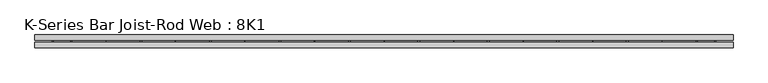
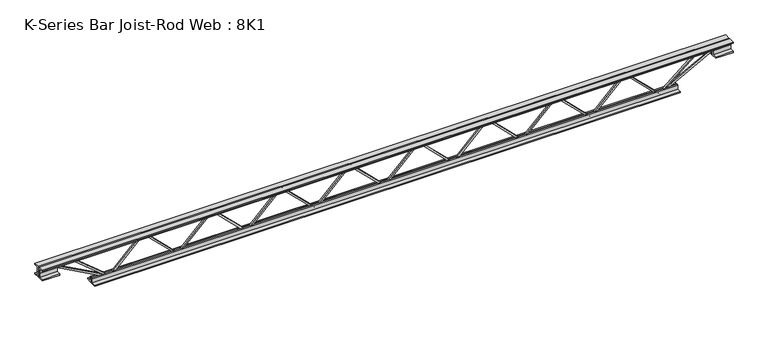
"""IFC4 building model written with IfcOpenShell, lengths in millimetres: beam geometry, K-Series Bar Joist-Rod Web : 8K1."""

from ifc_helpers import new_model, si_unit, frame, origin, place, context, project, spatial, polyline, outline, extrude, source, transform, mapped, element, save


def k_series_bar_joist_rod_web_8k1_7126daa4(model_context):
    return source(origin(), model_context, "Body", "SweptSolid", [
        extrude(outline(polyline([(-90.4875, 796.4251012), (-100.0125, 796.4251012), (-100.0125, 801.5563895), (90.4875, 994.3126648), (90.4875, 996.7500882), (-100.0125, 1189.5063635), (-100.0125, 1194.6376518), (-90.4875, 1194.6376518), (-90.4875, 1193.4189401), (100.0125, 1000.6626648), (100.0125, 990.4000882), (-90.4875, 797.6438129), (-90.4875, 796.4251012)])), frame((0.0, -4.7625, 0.0), z_axis=(0.0, 1.0, 0.0), x_axis=(0.0, 0.0, 1.0)), (0.0, 0.0, 1.0), 9.525),
        extrude(outline(polyline([(-90.4875, 398.2125506), (-100.0125, 398.2125506), (-100.0125, 403.3438389), (90.4875, 596.1001142), (90.4875, 598.5375376), (-100.0125, 791.2938129), (-100.0125, 796.4251012), (-90.4875, 796.4251012), (-90.4875, 795.2063895), (100.0125, 602.4501142), (100.0125, 592.1875376), (-90.4875, 399.4312623), (-90.4875, 398.2125506)])), frame((0.0, -4.7625, 0.0), z_axis=(0.0, 1.0, 0.0), x_axis=(0.0, 0.0, 1.0)), (0.0, 0.0, 1.0), 9.525),
        extrude(outline(polyline([(-90.4875, 0.0), (-100.0125, 0.0), (-100.0125, 5.1312883), (90.4875, 197.8875636), (90.4875, 200.324987), (-100.0125, 393.0812623), (-100.0125, 398.2125506), (-90.4875, 398.2125506), (-90.4875, 396.9938389), (100.0125, 204.2375636), (100.0125, 193.974987), (-90.4875, 1.2187117), (-90.4875, 0.0)])), frame((0.0, -4.7625, 0.0), z_axis=(0.0, 1.0, 0.0), x_axis=(0.0, 0.0, 1.0)), (0.0, 0.0, 1.0), 9.525),
        extrude(outline(polyline([(-90.4875, -398.2125506), (-100.0125, -398.2125506), (-100.0125, -393.0812623), (90.4875, -200.324987), (90.4875, -197.8875636), (-100.0125, -5.1312883), (-100.0125, 0.0), (-90.4875, 0.0), (-90.4875, -1.2187117), (100.0125, -193.974987), (100.0125, -204.2375636), (-90.4875, -396.9938389), (-90.4875, -398.2125506)])), frame((0.0, -4.7625, 0.0), z_axis=(0.0, 1.0, 0.0), x_axis=(0.0, 0.0, 1.0)), (0.0, 0.0, 1.0), 9.525),
        extrude(outline(polyline([(-90.4875, -796.4251012), (-100.0125, -796.4251012), (-100.0125, -791.2938129), (90.4875, -598.5375376), (90.4875, -596.1001142), (-100.0125, -403.3438389), (-100.0125, -398.2125506), (-90.4875, -398.2125506), (-90.4875, -399.4312623), (100.0125, -592.1875376), (100.0125, -602.4501142), (-90.4875, -795.2063895), (-90.4875, -796.4251012)])), frame((0.0, -4.7625, 0.0), z_axis=(0.0, 1.0, 0.0), x_axis=(0.0, 0.0, 1.0)), (0.0, 0.0, 1.0), 9.525),
        extrude(outline(polyline([(-90.4875, -1194.6376518), (-100.0125, -1194.6376518), (-100.0125, -1189.5063635), (90.4875, -996.7500882), (90.4875, -994.3126648), (-100.0125, -801.5563895), (-100.0125, -796.4251012), (-90.4875, -796.4251012), (-90.4875, -797.6438129), (100.0125, -990.4000882), (100.0125, -1000.6626648), (-90.4875, -1193.4189401), (-90.4875, -1194.6376518)])), frame((0.0, -4.7625, 0.0), z_axis=(0.0, 1.0, 0.0), x_axis=(0.0, 0.0, 1.0)), (0.0, 0.0, 1.0), 9.525),
        extrude(outline(polyline([(-90.4875, 1194.6376518), (-100.0125, 1194.6376518), (-100.0125, 1199.7689401), (90.4875, 1392.5252154), (90.4875, 1394.9626388), (-100.0125, 1587.7189141), (-100.0125, 1592.8502024), (-90.4875, 1592.8502024), (-90.4875, 1591.6314907), (100.0125, 1398.8752154), (100.0125, 1388.6126388), (-90.4875, 1195.8563635), (-90.4875, 1194.6376518)])), frame((0.0, -4.7625, 0.0), z_axis=(0.0, 1.0, 0.0), x_axis=(0.0, 0.0, 1.0)), (0.0, 0.0, 1.0), 9.525),
        extrude(outline(polyline([(-90.4875, -1592.8502024), (-100.0125, -1592.8502024), (-100.0125, -1587.7189141), (90.4875, -1394.9626388), (90.4875, -1392.5252154), (-100.0125, -1199.7689401), (-100.0125, -1194.6376518), (-90.4875, -1194.6376518), (-90.4875, -1195.8563635), (100.0125, -1388.6126388), (100.0125, -1398.8752154), (-90.4875, -1591.6314907), (-90.4875, -1592.8502024)])), frame((0.0, -4.7625, 0.0), z_axis=(0.0, 1.0, 0.0), x_axis=(0.0, 0.0, 1.0)), (0.0, 0.0, 1.0), 9.525),
        extrude(outline(polyline([(4.7625, 101.6), (36.5125, 101.6), (36.5125, 95.25), (11.1125, 95.25), (11.1125, 69.85), (4.7625, 69.85), (4.7625, 101.6)])), frame((-1999.2502024, 0.0, 0.0), z_axis=(1.0, 0.0, 0.0), x_axis=(0.0, 1.0, 0.0)), (0.0, 0.0, 1.0), 3998.5004049),
        extrude(outline(polyline([(-4.7625, 101.6), (-4.7625, 69.85), (-11.1125, 69.85), (-11.1125, 95.25), (-36.5125, 95.25), (-36.5125, 101.6), (-4.7625, 101.6)])), frame((-1999.2502024, 0.0, 0.0), z_axis=(1.0, 0.0, 0.0), x_axis=(0.0, 1.0, 0.0)), (0.0, 0.0, 1.0), 3998.5004049),
        extrude(outline(polyline([(-4.7625, 38.1), (-36.5125, 38.1), (-36.5125, 44.45), (-11.1125, 44.45), (-11.1125, 69.85), (-4.7625, 69.85), (-4.7625, 38.1)])), frame((-1999.2502024, 0.0, 0.0), z_axis=(1.0, 0.0, 0.0), x_axis=(0.0, 1.0, 0.0)), (0.0, 0.0, 1.0), 101.6),
        extrude(outline(polyline([(36.5125, 38.1), (4.7625, 38.1), (4.7625, 69.85), (11.1125, 69.85), (11.1125, 44.45), (36.5125, 44.45), (36.5125, 38.1)])), frame((-1999.2502024, 0.0, 0.0), z_axis=(1.0, 0.0, 0.0), x_axis=(0.0, 1.0, 0.0)), (0.0, 0.0, 1.0), 101.6),
        extrude(outline(polyline([(4.7625, 38.1), (4.7625, 69.85), (11.1125, 69.85), (11.1125, 44.45), (36.5125, 44.45), (36.5125, 38.1), (4.7625, 38.1)])), frame((1897.6502024, 0.0, 0.0), z_axis=(1.0, 0.0, 0.0), x_axis=(0.0, 1.0, 0.0)), (0.0, 0.0, 1.0), 101.6),
        extrude(outline(polyline([(-4.7625, 38.1), (-36.5125, 38.1), (-36.5125, 44.45), (-11.1125, 44.45), (-11.1125, 69.85), (-4.7625, 69.85), (-4.7625, 38.1)])), frame((1897.6502024, 0.0, 0.0), z_axis=(1.0, 0.0, 0.0), x_axis=(0.0, 1.0, 0.0)), (0.0, 0.0, 1.0), 101.6),
        extrude(outline(polyline([(4.7625, -101.6), (4.7625, -69.85), (11.1125, -69.85), (11.1125, -95.25), (36.5125, -95.25), (36.5125, -101.6), (4.7625, -101.6)])), frame((-1694.4502024, 0.0, 0.0), z_axis=(1.0, 0.0, 0.0), x_axis=(0.0, 1.0, 0.0)), (0.0, 0.0, 1.0), 3388.9004049),
        extrude(outline(polyline([(-4.7625, -101.6), (-36.5125, -101.6), (-36.5125, -95.25), (-11.1125, -95.25), (-11.1125, -69.85), (-4.7625, -69.85), (-4.7625, -101.6)])), frame((-1694.4502024, 0.0, 0.0), z_axis=(1.0, 0.0, 0.0), x_axis=(0.0, 1.0, 0.0)), (0.0, 0.0, 1.0), 3388.9004049),
        extrude(outline(polyline([(0.0, -9.525), (0.0, 0.0), (346.6425392, 0.0), (346.6425392, -9.525), (0.0, -9.525)])), frame((-1899.9185009, 4.7625, 65.662372), z_axis=(0.47628314854008014, 0.0, 0.8792919665371384), x_axis=(0.8792919665371384, 0.0, -0.47628314854008014)), (0.0, 0.0, 1.0), 9.525),
        extrude(outline(polyline([(0.0, -9.525), (0.0, 0.0), (258.6528926, 0.0), (258.6528926, -9.525), (0.0, -9.525)])), frame((-1794.9964157, 4.7625, 66.1839144), z_axis=(0.6383071858239102, 0.0, 0.769781746032965), x_axis=(0.769781746032965, 0.0, -0.6383071858239102)), (0.0, 0.0, 1.0), 9.525),
        extrude(outline(polyline([(0.0, -9.525), (0.0, 0.0), (346.6425392, 0.0), (346.6425392, -9.525), (0.0, -9.525)])), frame((1899.9185009, -4.7625, 65.662372), z_axis=(-0.47628314854004167, 0.0, 0.8792919665371591), x_axis=(-0.8792919665371591, 0.0, -0.47628314854004167)), (0.0, 0.0, 1.0), 9.525),
        extrude(outline(polyline([(0.0, -9.525), (0.0, 0.0), (258.6528926, 0.0), (258.6528926, -9.525), (0.0, -9.525)])), frame((1794.9964157, -4.7625, 66.1839144), z_axis=(-0.6383071858238841, 0.0, 0.7697817460329867), x_axis=(-0.7697817460329867, 0.0, -0.6383071858238841)), (0.0, 0.0, 1.0), 9.525),
    ])


if __name__ == "__main__":
    model = new_model("IFC4")
    model_context = context("Model", 3, world=origin())
    ifc_project = project(units=[si_unit("LENGTHUNIT", "METRE", prefix="MILLI")], contexts=[model_context])
    site = spatial("IfcSite", under=ifc_project)
    building = spatial("IfcBuilding", under=site)
    placement = place(None, origin())
    k_series_bar_joist_rod_web_8k1_shape = k_series_bar_joist_rod_web_8k1_7126daa4(model_context)
    element("IfcBeam", 1, ObjectType="K-Series Bar Joist-Rod Web : 8K1", at=placement, inside=building, context=model_context, shape_type="MappedRepresentation", body=[
        mapped(k_series_bar_joist_rod_web_8k1_shape, transform((0.0, 0.0, 0.0), x_axis=(1.0, 0.0, 0.0), y_axis=(0.0, 1.0, 0.0), z_axis=(0.0, 0.0, 1.0))),
    ])
    save(model, "model.ifc")

# Revit data of these elements
# Type "K-Series Bar Joist-Rod Web : 8K1"
#   Assembly Code = "B1010350"
#   Wt = 5.1
#   Web Thickness = 0' - 0 3/8"
#   Start Offset [instance default] = 0' - 0"
#   Start Extension [instance default] = 0' - 0"
#   Seat Length = 0' - 4"
#   Seat Depth = 0' - 2 1/2"
#   PanelArrayLength [instance default] = 21' - 4"
#   Panel [instance default] = 1' - 4"
#   End Offset [instance default] = 0' - 0"
#   End Extension [instance default] = 0' - 0"
#   End Panel = 1' - 4"
#   Cord Leg = 0' - 1 1/4"
#   Chord Thickness = 0' - 0 1/4"
#   Length [instance default] = 24' - 0"
#   Depth = 0' - 8"
#   PanelArrayNum [instance default] = 16
#   Rendering Material = none
# Element 1 (IfcBeam, "K-Series Bar Joist-Rod Web : 8K1")
#   PanelArrayLength = 10' - 5.42128"
#   Panel = 1' - 3.67766"
#   PanelArrayNum = 8
